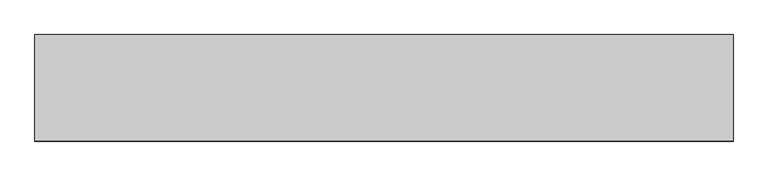
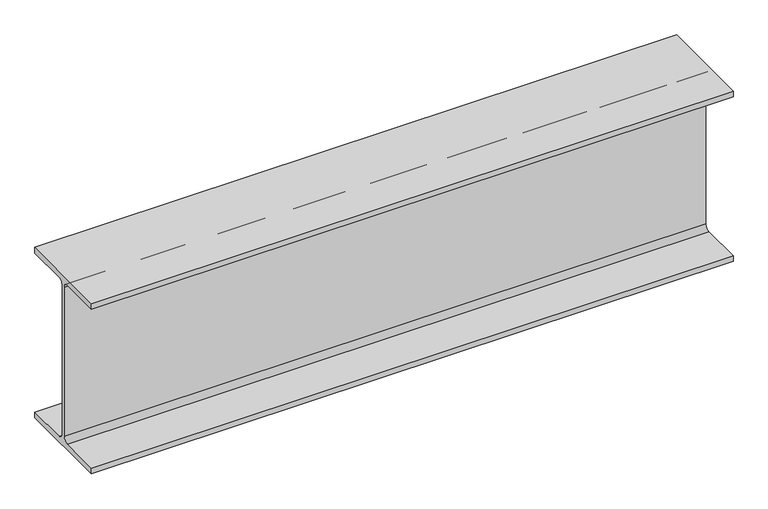
"""IFC4 building model written with IfcOpenShell, lengths in millimetres: beam geometry, Old_Steel Beam_H-KSD3502 : H_SB_ASB_H-482×300x11x15."""

from ifc_helpers import new_model, si_unit, point, frame, frame_2d, origin, place, context, project, spatial, polyline, circle_curve, trimmed, segment, composite_curve, outline, extrude, source, transform, mapped, element, save


def beam_beb0eca4(model_context):
    return source(origin(), model_context, "Body", "SweptSolid", [
        extrude(outline(composite_curve([segment(polyline([(82.5, -141.5), (82.5, -151.7), (-82.5, -151.7), (-82.5, -141.5), (-11.9, -141.5)]), True, "CONTINUOUS"), segment(trimmed(circle_curve(frame_2d((-11.9, -132.6)), 8.9), [point((-11.9, -141.5))], [point((-3.0, -132.6))], True, "CARTESIAN"), True, "CONTINUOUS"), segment(polyline([(-3.0, -132.6), (-3.0, 132.6)]), True, "CONTINUOUS"), segment(trimmed(circle_curve(frame_2d((-11.9, 132.6)), 8.9), [point((-3.0, 132.6))], [point((-11.9, 141.5))], True, "CARTESIAN"), True, "CONTINUOUS"), segment(polyline([(-11.9, 141.5), (-82.5, 141.5), (-82.5, 151.7), (82.5, 151.7), (82.5, 141.5), (11.9, 141.5)]), True, "CONTINUOUS"), segment(trimmed(circle_curve(frame_2d((11.9, 132.6)), 8.9), [point((11.9, 141.5))], [point((3.0, 132.6))], True, "CARTESIAN"), True, "CONTINUOUS"), segment(polyline([(3.0, 132.6), (3.0, -132.6)]), True, "CONTINUOUS"), segment(trimmed(circle_curve(frame_2d((11.9, -132.6)), 8.9), [point((3.0, -132.6))], [point((11.9, -141.5))], True, "CARTESIAN"), True, "CONTINUOUS"), segment(polyline([(11.9, -141.5), (82.5, -141.5)]), True, "CONTINUOUS")], self_intersect=False)), frame((-540.5, 0.0, 0.0), z_axis=(1.0, 0.0, 0.0), x_axis=(0.0, 1.0, 0.0)), (0.0, 0.0, 1.0), 1081.0),
    ])


if __name__ == "__main__":
    model = new_model("IFC4")
    model_context = context("Model", 3, world=origin())
    ifc_project = project(units=[si_unit("LENGTHUNIT", "METRE", prefix="MILLI")], contexts=[model_context])
    site = spatial("IfcSite", under=ifc_project)
    building = spatial("IfcBuilding", under=site)
    placement = place(None, origin())
    beam_shape = beam_beb0eca4(model_context)
    element("IfcBeam", 1, ObjectType="Old_Steel Beam_H-KSD3502 : H_SB_ASB_H-482×300x11x15", at=placement, inside=building, context=model_context, shape_type="MappedRepresentation", body=[
        mapped(beam_shape, transform((0.0, 0.0, 0.0), x_axis=(1.0, 0.0, 0.0), y_axis=(0.0, 1.0, 0.0), z_axis=(0.0, 0.0, 1.0))),
    ])
    save(model, "model.ifc")

# Revit data of these elements
# Type "Old_Steel Beam_H-KSD3502 : H_SB_ASB_H-482×300x11x15"
#   Width = 30.0 cm
#   Web Thickness = 1.1 cm
#   Web Fillet = 2.6 cm
#   Warping Constant = 3680250.0 cm⁶
#   Torsional Moment of Inertia = 88.2192 cm⁴
#   Torsional Modulus = 1.0 cm³
#   Section Area = 145.5 cm²
#   Plastic Modulus weak axis = 695.0 cm³
#   Plastic Modulus strong axis = 2790.0 cm³
#   Perimeter = 2.10 m²/m
#   Nominal Weight = 114.00 kgf/m
#   Moment of Inertia weak axis = 6760.00 cm⁴
#   Moment of Inertia strong axis = 60400.00 cm⁴
#   Height = 48.2 cm
#   Flange Thickness = 1.5 cm
#   Elastic Modulus weak axis = 451.0 cm³
#   Elastic Modulus strong axis = 2500.0 cm³
#   Centroid Vertical = 24.1 cm
#   Centroid Horizontal = 15.0 cm
#   Length [instance default] = 1.5240 m
#   Structural Material [instance default] = Steel, 45-345
#   Assembly Code = ""
# Element 1 (IfcBeam, "Old_Steel Beam_H-KSD3502 : H_SB_ASB_H-482×300x11x15")
#   Structural Material = none
# Materials
#   "Steel, 45-345": class "Metal", colour RGB 189 187 185, transparency 0, Description = "Steel 345 MPa", Cost = 0
